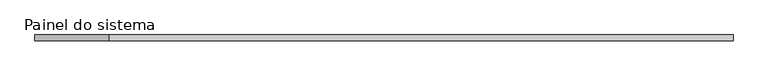
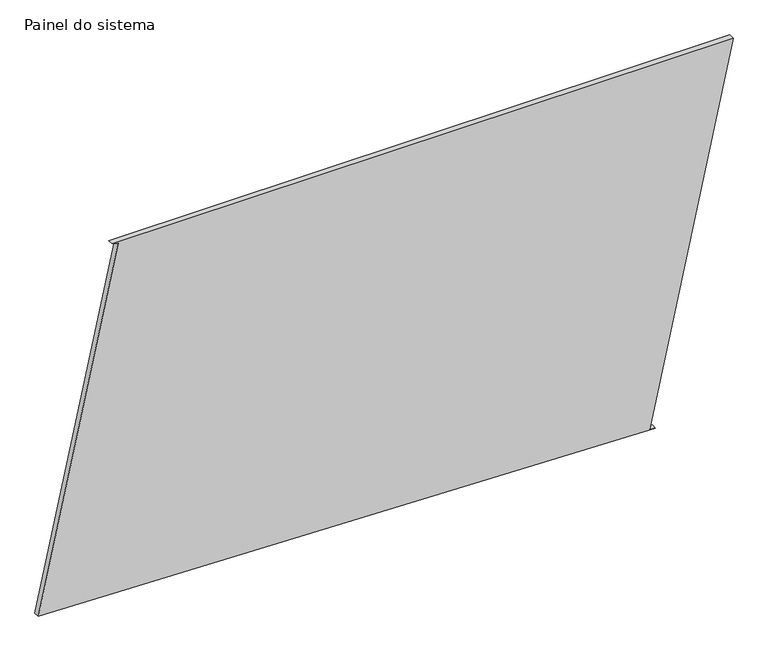
"""IFC4 building model written with IfcOpenShell, lengths in millimetres: plate geometry, Painel do sistema : Envidraçado."""

from ifc_helpers import new_model, si_unit, frame, origin, place, context, project, spatial, polyline, outline, extrude, source, transform, mapped, element, save


def painel_do_sistema_706a8e57(model_context):
    return source(origin(), model_context, "Body", "SweptSolid", [
        extrude(outline(polyline([(0.0, 1132.8033928), (5.3087357, 1108.3735479), (1617.2245381, 1458.651452), (1617.2245381, -1148.4352285), (1611.9158024, -1124.0053835), (71.9348913, -1458.651452), (0.0, 1132.8033928)])), frame((0.0, 24.5, 0.0), z_axis=(0.0, 1.0, 0.0), x_axis=(0.0, 0.0, 1.0)), (0.0, 0.0, 1.0), 25.0),
    ])


if __name__ == "__main__":
    model = new_model("IFC4")
    model_context = context("Model", 3, world=origin())
    ifc_project = project(units=[si_unit("LENGTHUNIT", "METRE", prefix="MILLI")], contexts=[model_context])
    site = spatial("IfcSite", under=ifc_project)
    building = spatial("IfcBuilding", under=site)
    placement = place(None, origin())
    painel_do_sistema_shape = painel_do_sistema_706a8e57(model_context)
    element("IfcPlate", 1, ObjectType="Painel do sistema : Envidraçado", at=placement, inside=building, context=model_context, shape_type="MappedRepresentation", body=[
        mapped(painel_do_sistema_shape, transform((0.0, 0.0, 0.0), x_axis=(1.0, 0.0, 0.0), y_axis=(0.0, 1.0, 0.0), z_axis=(0.0, 0.0, 1.0))),
    ])
    save(model, "model.ifc")

# Revit data of these elements
# Type "Painel do sistema : Envidraçado"
#   Construction Type Id = "GSP4R"
#   Analytic Construction = "Vidraça única Pilkington 1/8 pol"
#   Visual Light Transmittance = 0.9
#   Solar Heat Gain Coefficient = 0.86
#   Heat Transfer Coefficient (U) = 6.7069 W/(m²·K)
# Element 1 (IfcPlate, "Painel do sistema : Envidraçado")
#   Materials on its faces: "Vidro"
# Materials
#   "Vidro": class "Vidro", colour RGB 0 128 192, transparency 0.9, Description = "Vidro de sílica", Cost = 0
